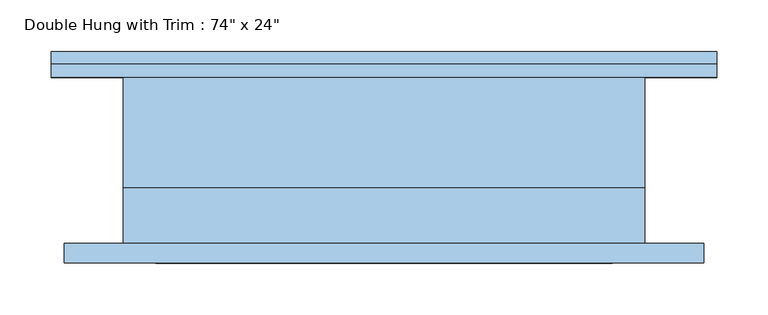
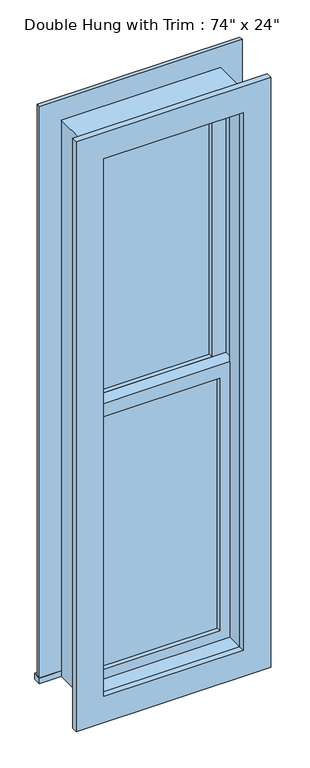
"""IFC4 building model written with IfcOpenShell, lengths in millimetres: window geometry."""

from ifc_helpers import new_model, si_unit, frame, origin, place, context, project, spatial, polyline, outline, extrude, source, transform, mapped, element, save


def window_84ecd6d1(model_context):
    return source(origin(), model_context, "Body", "SweptSolid", [
        extrude(outline(polyline([(-190.5, 1.5875), (190.5, 1.5875), (190.5, -11.1125), (-190.5, -11.1125), (-190.5, 1.5875)])), frame((0.0, 0.0, 673.1), z_axis=(0.0, 0.0, 1.0), x_axis=(1.0, 0.0, 0.0)), (0.0, 0.0, 1.0), 854.075),
        extrude(outline(polyline([(1571.625, -234.95), (628.65, -234.95), (628.65, 234.95), (1571.625, 234.95), (1571.625, -234.95)]), holes=[polyline([(1527.175, -190.5), (1527.175, 190.5), (673.1, 190.5), (673.1, -190.5), (1527.175, -190.5)])]), frame((0.0, -26.9875, 0.0), z_axis=(0.0, 1.0, 0.0), x_axis=(0.0, 0.0, 1.0)), (0.0, 0.0, 1.0), 44.45),
        extrude(outline(polyline([(-323.85, 106.3625), (323.85, 106.3625), (323.85, 80.9625), (-323.85, 80.9625), (-323.85, 106.3625)])), frame((0.0, 0.0, 609.6), z_axis=(0.0, 0.0, 1.0), x_axis=(1.0, 0.0, 0.0)), (0.0, 0.0, 1.0), 19.05),
        extrude(outline(polyline([(2470.15, -234.95), (2470.15, 234.95), (628.65, 234.95), (628.65, 323.85), (2559.05, 323.85), (2559.05, -323.85), (628.65, -323.85), (628.65, -234.95), (2470.15, -234.95)])), frame((0.0, 80.9625, 0.0), z_axis=(0.0, 1.0, 0.0), x_axis=(0.0, 0.0, 1.0)), (0.0, 0.0, 1.0), 12.7),
        extrude(outline(polyline([(2546.35, 311.15), (2546.35, -311.15), (552.45, -311.15), (552.45, 311.15), (2546.35, 311.15)]), holes=[polyline([(2457.45, 222.25), (641.35, 222.25), (641.35, -222.25), (2457.45, -222.25), (2457.45, 222.25)])]), frame((0.0, -100.0125, 0.0), z_axis=(0.0, 1.0, 0.0), x_axis=(0.0, 0.0, 1.0)), (0.0, 0.0, 1.0), 19.05),
        extrude(outline(polyline([(190.5, 33.3375), (-190.5, 33.3375), (-190.5, 46.0375), (190.5, 46.0375), (190.5, 33.3375)])), frame((0.0, 0.0, 1571.625), z_axis=(0.0, 0.0, 1.0), x_axis=(1.0, 0.0, 0.0)), (0.0, 0.0, 1.0), 854.075),
        extrude(outline(polyline([(2470.15, -234.95), (1527.175, -234.95), (1527.175, 234.95), (2470.15, 234.95), (2470.15, -234.95)]), holes=[polyline([(2425.7, -190.5), (2425.7, 190.5), (1571.625, 190.5), (1571.625, -190.5), (2425.7, -190.5)])]), frame((0.0, 17.4625, 0.0), z_axis=(0.0, 1.0, 0.0), x_axis=(0.0, 0.0, 1.0)), (0.0, 0.0, 1.0), 44.45),
        extrude(outline(polyline([(2489.2, -254.0), (609.6, -254.0), (609.6, 254.0), (2489.2, 254.0), (2489.2, -254.0)]), holes=[polyline([(2457.45, -222.25), (2457.45, 222.25), (641.35, 222.25), (641.35, -222.25), (2457.45, -222.25)])]), frame((0.0, -80.9625, 0.0), z_axis=(0.0, 1.0, 0.0), x_axis=(0.0, 0.0, 1.0)), (0.0, 0.0, 1.0), 53.975),
        extrude(outline(polyline([(2489.2, 254.0), (2489.2, -254.0), (609.6, -254.0), (609.6, 254.0), (2489.2, 254.0)]), holes=[polyline([(2470.15, 234.95), (628.65, 234.95), (628.65, -234.95), (2470.15, -234.95), (2470.15, 234.95)])]), frame((0.0, -26.9875, 0.0), z_axis=(0.0, 1.0, 0.0), x_axis=(0.0, 0.0, 1.0)), (0.0, 0.0, 1.0), 107.95),
    ])


if __name__ == "__main__":
    model = new_model("IFC4")
    model_context = context("Model", 3, world=origin())
    ifc_project = project(units=[si_unit("LENGTHUNIT", "METRE", prefix="MILLI")], contexts=[model_context])
    site = spatial("IfcSite", under=ifc_project)
    building = spatial("IfcBuilding", under=site)
    placement = place(None, origin())
    window_shape = window_84ecd6d1(model_context)
    element("IfcWindow", 1, ObjectType="Double Hung with Trim : 74\" x 24\"", at=placement, inside=building, context=model_context, shape_type="MappedRepresentation", body=[
        mapped(window_shape, transform((0.0, 0.0, 0.0), x_axis=(1.0, 0.0, 0.0), y_axis=(0.0, 1.0, 0.0), z_axis=(0.0, 0.0, 1.0))),
    ])
    save(model, "model.ifc")

# Revit data of these elements
# Type "Double Hung with Trim : 74\" x 24\""
#   Type Mark = "63"
#   COBie.Type.CreatedBy = "doug.wood@us.ibm.com"
#   COBie.Type.CreatedOn = "2016-04-14T02:07:26"
#   COBie.Type.Name = "Windows_Double Hung with Trim_74\" x 24\"_63"
#   COBie.Type.Category = "23-30 20 17 17 14 : Double-Hung Windows"
#   COBie.Type.Description = "Double Hung with Trim_74\" x 24\""
#   COBie.Type.Manufacturer = ""
#   COBie.Type.ModelNumber = ""
#   Construction Type Id = "GSP4R"
#   Assembly Code = "B2020100"
#   Analytic Construction = "1/8 in Pilkington single glazing"
#   COBie.Type.ReplacementCost = 0
#   Visual Light Transmittance = 0.9
#   Solar Heat Gain Coefficient = 0.78
#   Heat Transfer Coefficient (U) = 3.6886 W/(m²·K)
#   Height = 6' - 2"
#   Default Sill Height = 2' - 0"
#   Trim Projection - Ext. = 0' - 0 1/2"
#   Trim Projection - Int. = 0' - 0 3/4"
#   Trim Width - Exterior = 0' - 3 1/2"
#   Trim Width - Interior = 0' - 3 1/2"
#   Width = 1' - 8"
#   Window Inset = 0' - 0 3/4"
#   COBie.Type = no
#   Glass Pane Material = Glass
#   Sash Material = Sash - White
#   Trim Exterior Material = Trim - White
#   Trim Interior Material = Trim - White
#   Wall Closure = (empty or 0)
# Element 1 (IfcWindow, "Double Hung with Trim : 74\" x 24\"")
#   Materials on its faces: "Sash - White", "Trim - White", "Glass"
# Materials
#   "Glass": class "Glass", colour RGB 0 128 192, transparency 0.75, Description = "Soda Lime Glass", Cost = 0
#   "Sash - White": class "Wood", colour RGB 255 255 255, transparency 0, Cost = 0
#   "Trim - White": class "Wood", colour RGB 255 255 255, transparency 0, Cost = 0
